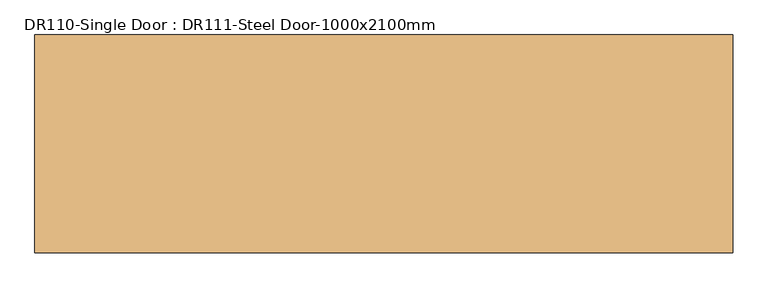
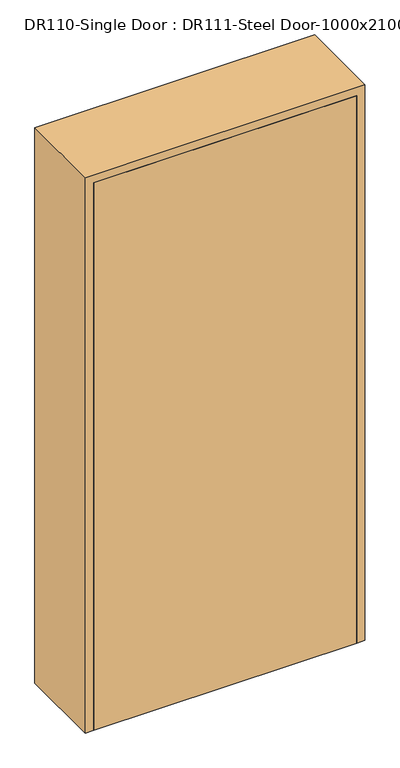
"""IFC4 building model written with IfcOpenShell, lengths in millimetres: door geometry, DR110-Single Door : DR111-Steel Door-1000x2100mm."""

from ifc_helpers import new_model, si_unit, origin, origin_with_axes, place, context, project, spatial, polyline, outline, extrude, faceted_brep, source, transform, mapped, element, save


def dr110_single_door_dr111_steel_door_1000x2100mm_363572d3(model_context):
    return source(origin(), model_context, "Body", "SolidModel", [
        extrude(outline(polyline([(470.0, -156.0), (-470.0, -156.0), (-470.0, -121.0), (470.0, -121.0), (470.0, -156.0)])), origin_with_axes(), (0.0, 0.0, 1.0), 2070.0),
        faceted_brep([(470.0, -156.0, 0.0), (470.0, -121.0, 0.0), (450.0, -121.0, 0.0), (450.0, 121.0, 0.0), (470.0, 121.0, 0.0), (470.0, 156.0, 0.0), (500.0, 156.0, 0.0), (500.0, -156.0, 0.0), (500.0, -156.0, 2100.0), (-500.0, -156.0, 2100.0), (-500.0, -156.0, 0.0), (-470.0, -156.0, 0.0), (-470.0, -156.0, 2070.0), (470.0, -156.0, 2070.0), (500.0, 156.0, 2100.0), (470.0, 156.0, 2070.0), (-470.0, 156.0, 2070.0), (-470.0, 156.0, 0.0), (-500.0, 156.0, 0.0), (-500.0, 156.0, 2100.0), (470.0, 121.0, 2070.0), (450.0, 121.0, 2050.0), (-450.0, 121.0, 2050.0), (-450.0, 121.0, 0.0), (-470.0, 121.0, 0.0), (-470.0, 121.0, 2070.0), (450.0, -121.0, 2050.0), (470.0, -121.0, 2070.0), (-470.0, -121.0, 2070.0), (-470.0, -121.0, 0.0), (-450.0, -121.0, 0.0), (-450.0, -121.0, 2050.0)], [[[0, 1, 2, 3, 4, 5, 6, 7]], [[7, 8, 9, 10, 11, 12, 13, 0]], [[6, 14, 8, 7]], [[5, 15, 16, 17, 18, 19, 14, 6]], [[4, 20, 15, 5]], [[3, 21, 22, 23, 24, 25, 20, 4]], [[2, 26, 21, 3]], [[1, 27, 28, 29, 30, 31, 26, 2]], [[0, 13, 27, 1]], [[12, 11, 29, 28]], [[11, 10, 18, 17, 24, 23, 30, 29]], [[19, 18, 10, 9]], [[25, 24, 17, 16]], [[31, 30, 23, 22]], [[14, 19, 9, 8]], [[20, 25, 16, 15]], [[26, 31, 22, 21]], [[13, 12, 28, 27]]]),
    ])


if __name__ == "__main__":
    model = new_model("IFC4")
    model_context = context("Model", 3, world=origin())
    ifc_project = project(units=[si_unit("LENGTHUNIT", "METRE", prefix="MILLI")], contexts=[model_context])
    site = spatial("IfcSite", under=ifc_project)
    building = spatial("IfcBuilding", under=site)
    placement = place(None, origin())
    dr110_single_door_dr111_steel_door_1000x2100mm_shape = dr110_single_door_dr111_steel_door_1000x2100mm_363572d3(model_context)
    element("IfcDoor", 1, ObjectType="DR110-Single Door : DR111-Steel Door-1000x2100mm", at=placement, inside=building, context=model_context, shape_type="MappedRepresentation", body=[
        mapped(dr110_single_door_dr111_steel_door_1000x2100mm_shape, transform((0.0, 0.0, 0.0), x_axis=(1.0, 0.0, 0.0), y_axis=(0.0, 1.0, 0.0), z_axis=(0.0, 0.0, 1.0))),
    ])
    save(model, "model.ifc")

# Revit data of these elements
# Type "DR110-Single Door : DR111-Steel Door-1000x2100mm"
#   Description = "DSDSSD"
#   Type Mark = "SD"
#   Analytic Construction = "<None>"
#   프레임 투영 외부. = 25 mm
#   프레임 투영 내부. = 25 mm
#   프레임 폭 = 75 mm
#   Height = 2100 mm
#   Width = 1000 mm
#   Define Thermal Properties by = 1
#   문 패널 = SD1 문 패널
#   문 프레임 = A04AQ098-00002_Steel Door_non FP_single
#   Function = (empty or 0)
#   Wall Closure = (empty or 0)
# Element 1 (IfcDoor, "DR110-Single Door : DR111-Steel Door-1000x2100mm")
#   Materials on its faces: "A04AQ098-00002_Steel Door_non FP_single", "SD1 문 패널"
# Materials
#   "SD1 문 패널": class "금속", colour RGB 247 247 247, transparency 0, Description = "STEEL DOOR (1000Wx2100H)"
#   "A04AQ098-00002_Steel Door_non FP_single": class "금속", colour RGB 247 247 247, transparency 0, Description = "Steel Door", W00) Work Master Code = "A04AQ098-00002", W01) Work Master_Lv1 = "Finishing Work", W02) Work Master_Lv2 = "Door & Window Work", W03) Work Master_Spec.1 = "Steel Door w/ Steel Frame", W04) Work Master_Spec.2 = "Fire Protective Rating: N/A, Single Door", W05) Work Master_Spec.3 = "w/ Hardware & Accessories", Cost = 0
